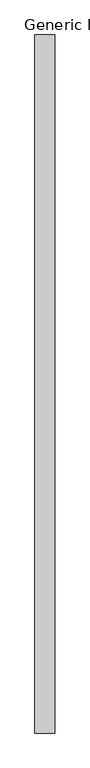
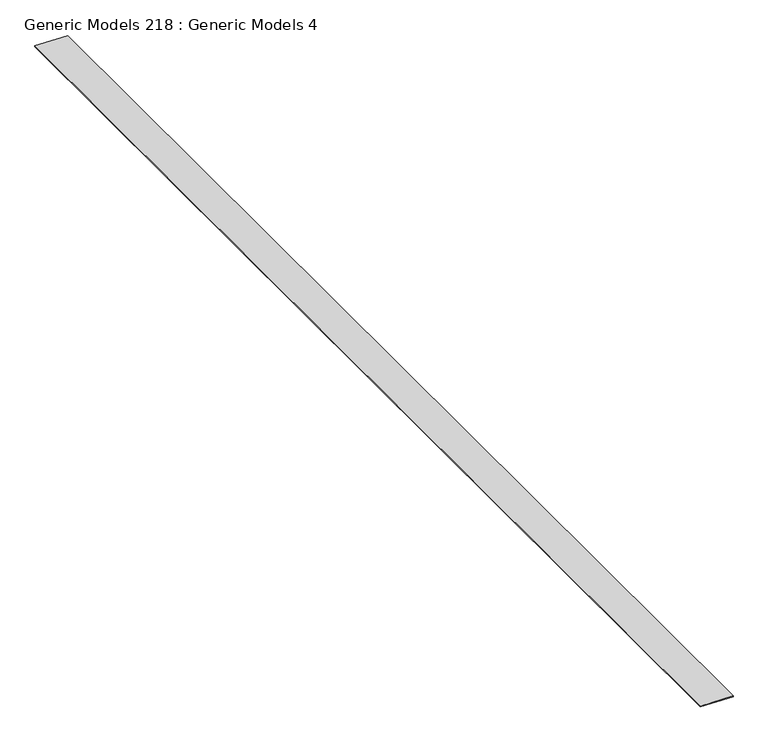
"""IFC4 building model written with IfcOpenShell, lengths in millimetres: proxy geometry, Generic Models 218 : Generic Models 4."""

import ifcopenshell
import ifcopenshell.guid

model = None  # the IFC model being written
_history = None  # IfcOwnerHistory: only IFC2X3 demands one
_inside = {}  # id of a spatial element -> (the spatial element, [elements in it])
_under = {}  # id of a project, library or spatial element -> (it, [spatial elements below it])
_declared = {}  # id of a project -> (the project, [libraries it declares])
_typed = {}  # id of a type object -> (the type object, [elements of that type])
_made_of = {}  # id of a material, layer set ... -> (it, [elements and type objects made of it])


def new_model(schema):
    """Start an empty IFC model of exactly this schema.

    Asked for "IFC4X3", IfcOpenShell would pick the latest addendum, in which some entities
    have other attributes; the version numbers below select the first issue.
    IFC2X3 requires an IfcOwnerHistory on every rooted entity: one is made here for all.
    """
    global model, _history
    if schema == "IFC4X3":
        model = ifcopenshell.file(schema_version=(4, 3, 0, 0))
    else:
        model = ifcopenshell.file(schema=schema)
    _inside.clear()
    _under.clear()
    _declared.clear()
    _typed.clear()
    _made_of.clear()
    _history = None
    if model.schema == "IFC2X3":
        org = make("IfcOrganization", Name="unknown")
        user = make(
            "IfcPersonAndOrganization",
            ThePerson=make("IfcPerson", FamilyName="unknown"),
            TheOrganization=org,
        )
        app = make(
            "IfcApplication",
            ApplicationDeveloper=org,
            Version="unknown",
            ApplicationFullName="unknown",
            ApplicationIdentifier="unknown",
        )
        _history = make(
            "IfcOwnerHistory",
            OwningUser=user,
            OwningApplication=app,
            ChangeAction="ADDED",
            CreationDate=0,
        )
    return model


def make(cls, **values):
    """One entity of the class cls with the attributes given. An attribute that is None is left unset."""
    return model.create_entity(
        cls, **{name: value for name, value in values.items() if value is not None}
    )


def rooted(cls, **values):
    """An entity with a GlobalId (a new one), such as an element, a storey or a relation."""
    return make(cls, GlobalId=ifcopenshell.guid.new(), OwnerHistory=_history, **values)


def si_unit(unit_type, name, prefix=None):
    """IfcSIUnit, for example si_unit("LENGTHUNIT", "METRE", prefix="MILLI")."""
    return make("IfcSIUnit", UnitType=unit_type, Prefix=prefix, Name=name)


def assignment(units):
    """IfcUnitAssignment: the units of a project."""
    return None if units is None else make("IfcUnitAssignment", Units=units)


def point(xyz):
    """IfcCartesianPoint."""
    return None if xyz is None else make("IfcCartesianPoint", Coordinates=xyz)


def direction(xyz):
    """IfcDirection."""
    return None if xyz is None else make("IfcDirection", DirectionRatios=xyz)


def frame(location, z_axis=None, x_axis=None):
    """IfcAxis2Placement3D, a coordinate frame: its origin and axes. An axis left out is left unset."""
    return make(
        "IfcAxis2Placement3D",
        Location=point(location),
        Axis=direction(z_axis),
        RefDirection=direction(x_axis),
    )


def origin():
    """The frame at (0, 0, 0) with its axes left unset."""
    return frame((0.0, 0.0, 0.0))


def place(relative_to, where):
    """IfcLocalPlacement: puts the frame where relative to a parent placement (None: the world)."""
    return make(
        "IfcLocalPlacement", PlacementRelTo=relative_to, RelativePlacement=where
    )


def context(
    kind, dimensions, precision=None, world=None, true_north=None, identifier=None
):
    """IfcGeometricRepresentationContext, for example the 3D "Model" context."""
    return make(
        "IfcGeometricRepresentationContext",
        ContextIdentifier=identifier,
        ContextType=kind,
        CoordinateSpaceDimension=dimensions,
        Precision=precision,
        WorldCoordinateSystem=world,
        TrueNorth=true_north,
    )


def project(units=None, contexts=None):
    """IfcProject with its units and contexts."""
    return rooted(
        "IfcProject",
        Name="project",
        RepresentationContexts=contexts,
        UnitsInContext=assignment(units),
    )


def spatial(cls, under=None, at=None, **own):
    """A site, building, storey or space (cls), placed at a placement, below another one or the project."""
    s = rooted(cls, ObjectPlacement=at, **own)
    if under is not None:
        _under.setdefault(under.id(), (under, []))[1].append(s)
    return s


def polyline(points):
    """IfcPolyline through the points."""
    return make("IfcPolyline", Points=[point(p) for p in points])


def outline(outer, holes=None, kind="AREA"):
    """IfcArbitraryClosedProfileDef: a profile drawn as a closed curve; with holes, ...WithVoids."""
    if holes is None:
        return make("IfcArbitraryClosedProfileDef", ProfileType=kind, OuterCurve=outer)
    return make(
        "IfcArbitraryProfileDefWithVoids",
        ProfileType=kind,
        OuterCurve=outer,
        InnerCurves=holes,
    )


def extrude(swept, where, along, depth):
    """IfcExtrudedAreaSolid: the profile swept, set in the frame where, extruded along a direction by depth."""
    return make(
        "IfcExtrudedAreaSolid",
        SweptArea=swept,
        Position=where,
        ExtrudedDirection=direction(along),
        Depth=depth,
    )


def shape(context_of_items, identifier, shape_type, items):
    """IfcShapeRepresentation: the items that make up one representation, for example the "Body"."""
    return make(
        "IfcShapeRepresentation",
        ContextOfItems=context_of_items,
        RepresentationIdentifier=identifier,
        RepresentationType=shape_type,
        Items=items,
    )


def source(mapping_origin, context_of_items, identifier, shape_type, items):
    """IfcRepresentationMap: a shape defined once, which mapped items show again and again."""
    return make(
        "IfcRepresentationMap",
        MappingOrigin=mapping_origin,
        MappedRepresentation=shape(context_of_items, identifier, shape_type, items),
    )


def transform(
    local_origin,
    x_axis=None,
    y_axis=None,
    z_axis=None,
    scale=None,
    scale2=None,
    scale3=None,
    uniform=True,
):
    """IfcCartesianTransformationOperator3D, or its non-uniform kind. x_axis, y_axis, z_axis: its Axis1, 2, 3."""
    if uniform:
        return make(
            "IfcCartesianTransformationOperator3D",
            Axis1=direction(x_axis),
            Axis2=direction(y_axis),
            LocalOrigin=point(local_origin),
            Scale=scale,
            Axis3=direction(z_axis),
        )
    return make(
        "IfcCartesianTransformationOperator3DnonUniform",
        Axis1=direction(x_axis),
        Axis2=direction(y_axis),
        LocalOrigin=point(local_origin),
        Scale=scale,
        Axis3=direction(z_axis),
        Scale2=scale2,
        Scale3=scale3,
    )


def mapped(mapping_source, mapping_target):
    """IfcMappedItem: shows the shape of a source again, moved by a transform."""
    return make(
        "IfcMappedItem", MappingSource=mapping_source, MappingTarget=mapping_target
    )


def made_of(thing, what):
    """Note that an element or type object is made of a material, layer set ...; save() writes the relation."""
    if what is not None:
        _made_of.setdefault(what.id(), (what, []))[1].append(thing)
    return thing


def element(
    cls,
    number,
    at=None,
    inside=None,
    cuts=None,
    type_object=None,
    material=None,
    context=None,
    identifier="Body",
    shape_type=None,
    held_by="IfcProductDefinitionShape",
    body=None,
    shapes=None,
    **own,
):
    """One element of the class cls, such as IfcWall. Its Tag is "e" and its number.

    at: its placement. inside: the storey or other place that contains it. cuts: it is an
    opening in that element (IfcRelVoidsElement). A single representation is given by context,
    identifier, shape_type and body (its items); several are given by shapes. held_by: the class
    of the entity that holds the representations. save() writes the other relations.
    """
    e = rooted(cls, Tag="e%d" % number, ObjectPlacement=at, **own)
    if body is not None:
        shapes = [shape(context, identifier, shape_type, body)]
    if shapes is not None:
        e.Representation = make(held_by, Representations=shapes)
    if inside is not None:
        _inside.setdefault(inside.id(), (inside, []))[1].append(e)
    if cuts is not None:
        rooted(
            "IfcRelVoidsElement", RelatingBuildingElement=cuts, RelatedOpeningElement=e
        )
    if type_object is not None:
        _typed.setdefault(type_object.id(), (type_object, []))[1].append(e)
    return made_of(e, material)


def aggregate(whole, parts):
    """IfcRelAggregates: a whole, such as a stair, and the parts it consists of."""
    return rooted("IfcRelAggregates", RelatingObject=whole, RelatedObjects=parts)


def save(model, path):
    """Write the relations noted so far, then the file.

    IfcRelAggregates (storeys below a building ...), IfcRelContainedInSpatialStructure (elements
    in a storey), IfcRelDefinesByType, IfcRelAssociatesMaterial and IfcRelDeclares: one each for
    every whole, place, type object, material and project.
    """
    for whole, parts in _under.values():
        aggregate(whole, parts)
    for where, things in _inside.values():
        rooted(
            "IfcRelContainedInSpatialStructure",
            RelatedElements=things,
            RelatingStructure=where,
        )
    for kind, things in _typed.values():
        rooted("IfcRelDefinesByType", RelatedObjects=things, RelatingType=kind)
    for what, things in _made_of.values():
        rooted("IfcRelAssociatesMaterial", RelatedObjects=things, RelatingMaterial=what)
    for by, libraries in _declared.values():
        rooted("IfcRelDeclares", RelatingContext=by, RelatedDefinitions=libraries)
    model.write(path)


def generic_models_218_generic_models_4_3895cb72(model_context):
    return source(origin(), model_context, "Body", "SweptSolid", [
        extrude(outline(polyline([(0.0, -532.7341933), (0.0, 0.0), (18643.6, 0.0), (18643.6, -532.7341933), (0.0, -532.7341933)])), frame((7285.0150882, -6864.9230338, 126918.8275355), z_axis=(0.020828813681888794, 0.0, 0.9997830567281111), x_axis=(0.0, 1.0, 0.0)), (0.0, 0.0, 1.0), 12.7),
    ])


if __name__ == "__main__":
    model = new_model("IFC4")
    model_context = context("Model", 3, world=origin())
    ifc_project = project(units=[si_unit("LENGTHUNIT", "METRE", prefix="MILLI")], contexts=[model_context])
    site = spatial("IfcSite", under=ifc_project)
    building = spatial("IfcBuilding", under=site)
    placement = place(None, origin())
    generic_models_218_generic_models_4_shape = generic_models_218_generic_models_4_3895cb72(model_context)
    element("IfcBuildingElementProxy", 1, Name="Generic Models 218 : Generic Models 4", ObjectType="Generic Models 218 : Generic Models 4", at=placement, inside=building, context=model_context, shape_type="MappedRepresentation", body=[
        mapped(generic_models_218_generic_models_4_shape, transform((0.0, 0.0, 0.0), x_axis=(1.0, 0.0, 0.0), y_axis=(0.0, 1.0, 0.0), z_axis=(0.0, 0.0, 1.0))),
    ])
    save(model, "model.ifc")

# Revit data of these elements
# Element 1 (IfcBuildingElementProxy, "Generic Models 218 : Generic Models 4")
#   Materials on its faces: "_1/2\" CDX PLYWOOD"
# Materials
#   "_1/2\" CDX PLYWOOD": class "Generic", colour RGB 98 75 74, transparency 0, Cost = 0
